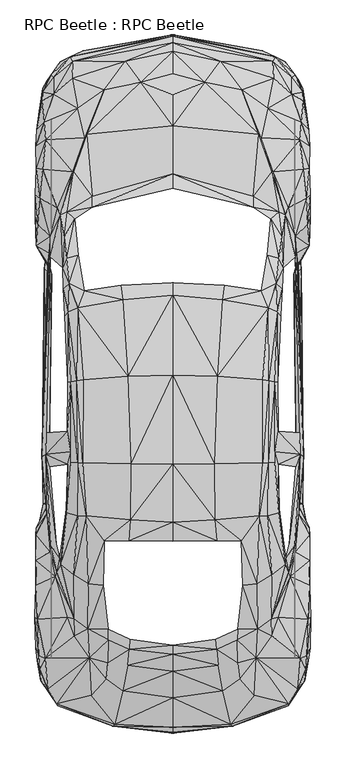
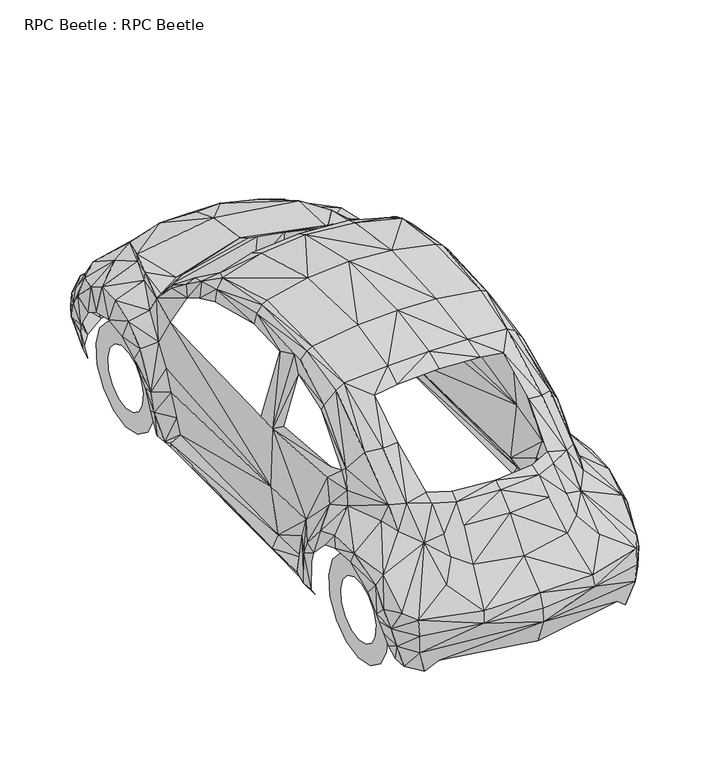
"""IFC4 building model written with IfcOpenShell, lengths in millimetres: proxy geometry, RPC Beetle : RPC Beetle."""

import ifcopenshell
import ifcopenshell.guid

model = None  # the IFC model being written
_history = None  # IfcOwnerHistory: only IFC2X3 demands one
_inside = {}  # id of a spatial element -> (the spatial element, [elements in it])
_under = {}  # id of a project, library or spatial element -> (it, [spatial elements below it])
_declared = {}  # id of a project -> (the project, [libraries it declares])
_typed = {}  # id of a type object -> (the type object, [elements of that type])
_made_of = {}  # id of a material, layer set ... -> (it, [elements and type objects made of it])


def new_model(schema):
    """Start an empty IFC model of exactly this schema.

    Asked for "IFC4X3", IfcOpenShell would pick the latest addendum, in which some entities
    have other attributes; the version numbers below select the first issue.
    IFC2X3 requires an IfcOwnerHistory on every rooted entity: one is made here for all.
    """
    global model, _history
    if schema == "IFC4X3":
        model = ifcopenshell.file(schema_version=(4, 3, 0, 0))
    else:
        model = ifcopenshell.file(schema=schema)
    _inside.clear()
    _under.clear()
    _declared.clear()
    _typed.clear()
    _made_of.clear()
    _history = None
    if model.schema == "IFC2X3":
        org = make("IfcOrganization", Name="unknown")
        user = make(
            "IfcPersonAndOrganization",
            ThePerson=make("IfcPerson", FamilyName="unknown"),
            TheOrganization=org,
        )
        app = make(
            "IfcApplication",
            ApplicationDeveloper=org,
            Version="unknown",
            ApplicationFullName="unknown",
            ApplicationIdentifier="unknown",
        )
        _history = make(
            "IfcOwnerHistory",
            OwningUser=user,
            OwningApplication=app,
            ChangeAction="ADDED",
            CreationDate=0,
        )
    return model


def make(cls, **values):
    """One entity of the class cls with the attributes given. An attribute that is None is left unset."""
    return model.create_entity(
        cls, **{name: value for name, value in values.items() if value is not None}
    )


def rooted(cls, **values):
    """An entity with a GlobalId (a new one), such as an element, a storey or a relation."""
    return make(cls, GlobalId=ifcopenshell.guid.new(), OwnerHistory=_history, **values)


def si_unit(unit_type, name, prefix=None):
    """IfcSIUnit, for example si_unit("LENGTHUNIT", "METRE", prefix="MILLI")."""
    return make("IfcSIUnit", UnitType=unit_type, Prefix=prefix, Name=name)


def assignment(units):
    """IfcUnitAssignment: the units of a project."""
    return None if units is None else make("IfcUnitAssignment", Units=units)


def point(xyz):
    """IfcCartesianPoint."""
    return None if xyz is None else make("IfcCartesianPoint", Coordinates=xyz)


def direction(xyz):
    """IfcDirection."""
    return None if xyz is None else make("IfcDirection", DirectionRatios=xyz)


def frame(location, z_axis=None, x_axis=None):
    """IfcAxis2Placement3D, a coordinate frame: its origin and axes. An axis left out is left unset."""
    return make(
        "IfcAxis2Placement3D",
        Location=point(location),
        Axis=direction(z_axis),
        RefDirection=direction(x_axis),
    )


def origin():
    """The frame at (0, 0, 0) with its axes left unset."""
    return frame((0.0, 0.0, 0.0))


def place(relative_to, where):
    """IfcLocalPlacement: puts the frame where relative to a parent placement (None: the world)."""
    return make(
        "IfcLocalPlacement", PlacementRelTo=relative_to, RelativePlacement=where
    )


def context(
    kind, dimensions, precision=None, world=None, true_north=None, identifier=None
):
    """IfcGeometricRepresentationContext, for example the 3D "Model" context."""
    return make(
        "IfcGeometricRepresentationContext",
        ContextIdentifier=identifier,
        ContextType=kind,
        CoordinateSpaceDimension=dimensions,
        Precision=precision,
        WorldCoordinateSystem=world,
        TrueNorth=true_north,
    )


def project(units=None, contexts=None):
    """IfcProject with its units and contexts."""
    return rooted(
        "IfcProject",
        Name="project",
        RepresentationContexts=contexts,
        UnitsInContext=assignment(units),
    )


def spatial(cls, under=None, at=None, **own):
    """A site, building, storey or space (cls), placed at a placement, below another one or the project."""
    s = rooted(cls, ObjectPlacement=at, **own)
    if under is not None:
        _under.setdefault(under.id(), (under, []))[1].append(s)
    return s


def point_list(points):
    """IfcCartesianPointList2D or 3D."""
    cls = (
        "IfcCartesianPointList2D" if len(points[0]) == 2 else "IfcCartesianPointList3D"
    )
    return make(cls, CoordList=points)


def triangles(points, corners, closed=None, point_numbers=None):
    """IfcTriangulatedFaceSet: each triangle names its three corners, points numbered from 1."""
    return make(
        "IfcTriangulatedFaceSet",
        Coordinates=point_list(points),
        Closed=closed,
        CoordIndex=corners,
        PnIndex=point_numbers,
    )


def shape(context_of_items, identifier, shape_type, items):
    """IfcShapeRepresentation: the items that make up one representation, for example the "Body"."""
    return make(
        "IfcShapeRepresentation",
        ContextOfItems=context_of_items,
        RepresentationIdentifier=identifier,
        RepresentationType=shape_type,
        Items=items,
    )


def source(mapping_origin, context_of_items, identifier, shape_type, items):
    """IfcRepresentationMap: a shape defined once, which mapped items show again and again."""
    return make(
        "IfcRepresentationMap",
        MappingOrigin=mapping_origin,
        MappedRepresentation=shape(context_of_items, identifier, shape_type, items),
    )


def transform(
    local_origin,
    x_axis=None,
    y_axis=None,
    z_axis=None,
    scale=None,
    scale2=None,
    scale3=None,
    uniform=True,
):
    """IfcCartesianTransformationOperator3D, or its non-uniform kind. x_axis, y_axis, z_axis: its Axis1, 2, 3."""
    if uniform:
        return make(
            "IfcCartesianTransformationOperator3D",
            Axis1=direction(x_axis),
            Axis2=direction(y_axis),
            LocalOrigin=point(local_origin),
            Scale=scale,
            Axis3=direction(z_axis),
        )
    return make(
        "IfcCartesianTransformationOperator3DnonUniform",
        Axis1=direction(x_axis),
        Axis2=direction(y_axis),
        LocalOrigin=point(local_origin),
        Scale=scale,
        Axis3=direction(z_axis),
        Scale2=scale2,
        Scale3=scale3,
    )


def mapped(mapping_source, mapping_target):
    """IfcMappedItem: shows the shape of a source again, moved by a transform."""
    return make(
        "IfcMappedItem", MappingSource=mapping_source, MappingTarget=mapping_target
    )


def made_of(thing, what):
    """Note that an element or type object is made of a material, layer set ...; save() writes the relation."""
    if what is not None:
        _made_of.setdefault(what.id(), (what, []))[1].append(thing)
    return thing


def element(
    cls,
    number,
    at=None,
    inside=None,
    cuts=None,
    type_object=None,
    material=None,
    context=None,
    identifier="Body",
    shape_type=None,
    held_by="IfcProductDefinitionShape",
    body=None,
    shapes=None,
    **own,
):
    """One element of the class cls, such as IfcWall. Its Tag is "e" and its number.

    at: its placement. inside: the storey or other place that contains it. cuts: it is an
    opening in that element (IfcRelVoidsElement). A single representation is given by context,
    identifier, shape_type and body (its items); several are given by shapes. held_by: the class
    of the entity that holds the representations. save() writes the other relations.
    """
    e = rooted(cls, Tag="e%d" % number, ObjectPlacement=at, **own)
    if body is not None:
        shapes = [shape(context, identifier, shape_type, body)]
    if shapes is not None:
        e.Representation = make(held_by, Representations=shapes)
    if inside is not None:
        _inside.setdefault(inside.id(), (inside, []))[1].append(e)
    if cuts is not None:
        rooted(
            "IfcRelVoidsElement", RelatingBuildingElement=cuts, RelatedOpeningElement=e
        )
    if type_object is not None:
        _typed.setdefault(type_object.id(), (type_object, []))[1].append(e)
    return made_of(e, material)


def aggregate(whole, parts):
    """IfcRelAggregates: a whole, such as a stair, and the parts it consists of."""
    return rooted("IfcRelAggregates", RelatingObject=whole, RelatedObjects=parts)


def save(model, path):
    """Write the relations noted so far, then the file.

    IfcRelAggregates (storeys below a building ...), IfcRelContainedInSpatialStructure (elements
    in a storey), IfcRelDefinesByType, IfcRelAssociatesMaterial and IfcRelDeclares: one each for
    every whole, place, type object, material and project.
    """
    for whole, parts in _under.values():
        aggregate(whole, parts)
    for where, things in _inside.values():
        rooted(
            "IfcRelContainedInSpatialStructure",
            RelatedElements=things,
            RelatingStructure=where,
        )
    for kind, things in _typed.values():
        rooted("IfcRelDefinesByType", RelatedObjects=things, RelatingType=kind)
    for what, things in _made_of.values():
        rooted("IfcRelAssociatesMaterial", RelatedObjects=things, RelatingMaterial=what)
    for by, libraries in _declared.values():
        rooted("IfcRelDeclares", RelatingContext=by, RelatedDefinitions=libraries)
    model.write(path)


def rpc_beetle_rpc_beetle_3ce7ba48(model_context):
    return source(origin(), model_context, "Body", "Tessellation", [
        triangles([(0.0, -748.5640469, 521.3893959), (0.0, -720.1452873, 603.6241656), (0.0, -696.6746996, 283.1362969), (0.0, -552.698168, 738.4050739), (0.0, -753.2493713, 438.4540149), (0.0, -253.6666567, 1039.7136446), (0.0, -401.102443, 921.3971746), (0.0, -304.8115909, 1012.258271), (0.0, 339.3168975, 1395.7139351), (0.0, 448.6129515, 1442.1297066), (0.0, 778.0774343, 1504.0465668), (0.0, 1285.0166222, 1509.4764679), (0.0, 1741.0736687, 1402.3260315), (0.0, 2430.9610645, 967.1999022), (0.0, 3130.000518, 632.0428888), (0.0, 3001.4374352, 771.5091579), (0.0, 2704.2451103, 928.7536297), (0.0, 3164.1993027, 220.1684652), (0.0, 2883.1647125, 858.7358105), (0.0, 3222.5253937, 395.8040382), (0.0, 3178.9995621, 555.7633515), (0.0, 3213.942778, 530.2784609), (-338.1784132, -715.5037102, 523.0095732), (-331.0408765, -702.1482754, 593.465229), (-244.7338081, -218.0228295, 1034.0649342), (-248.9812778, -275.9549947, 1002.9312967), (-257.7389736, -368.17353, 911.8512457), (-249.0688632, 342.8199903, 1381.001025), (-285.238149, -511.5369813, 760.4306917), (-240.1360146, 460.0855433, 1426.5848705), (-236.4577871, 780.8799522, 1493.4060825), (-652.4920767, -590.2248745, 370.4943186), (-540.0870918, -593.333878, 283.4428189), (-181.240518, 2954.2772324, 806.3210592), (-253.1849819, 1278.5798058, 1496.1646351), (-379.8650402, -444.3654636, 798.2639202), (-370.9321916, -353.3292326, 889.1688366), (-367.998359, -222.2265155, 1003.4567734), (-368.3924483, -160.7037083, 1036.6922447), (-390.1553278, 342.863774, 1359.0192272), (-282.5670547, 1713.2679531, 1399.3045589), (-397.3366482, 87.4893818, 1215.3492176), (-463.1069432, -537.7663033, 704.8193333), (-271.4885704, 3072.331073, 662.6947969), (-475.7618031, -323.0713775, 849.8467455), (-463.7199872, 3085.9052444, 214.2570165), (-482.2425121, 95.7654028, 1203.3949327), (-485.0449574, -159.3024857, 1005.0769506), (-568.7247334, 3071.4988564, 546.7429356), (-493.539933, 483.2496454, 1391.2912399), (-583.2625088, 3099.3922119, 522.0462235), (-510.267146, 3132.2774139, 369.3995816), (-391.8630724, 2911.6272194, 782.7628315), (-656.3454752, -597.8440679, 480.0968582), (-660.2426937, -584.8389024, 576.2563594), (-562.2878443, -200.0695467, 879.7105476), (-560.054623, -101.457906, 987.1674334), (-512.4565473, 786.1783207, 1448.435281), (-541.7948364, 484.782219, 1359.8511532), (-563.9955889, 148.5743069, 1172.3051153), (-608.4846974, -561.2369273, 218.4607206), (-511.2742793, 1258.5246346, 1456.1858253), (-542.4078804, 784.6895308, 1430.657151), (-458.8594554, 2304.0621243, 949.0276829), (-601.0406387, -92.7439938, 893.1973698), (-503.7426533, 1765.2887604, 1320.9670441), (-546.0423243, 1253.0072388, 1441.5166626), (-603.0111217, 501.1591264, 1278.5798058), (-580.1535416, 788.8931986, 1378.7239838), (-607.2148258, 519.8568223, 1235.1416142), (-601.2595934, 965.2732029, 1337.0374294), (-712.4823103, -503.0858256, 590.4876128), (-542.6706187, 1670.0487888, 1361.1648811), (-490.6061005, 2657.8729408, 893.5038918), (-599.6394161, 778.0774343, 1307.3049419), (-598.0630225, 1243.7240845, 1343.7807678), (-639.5744785, 208.1266312, 1062.483621), (-680.4291796, -470.2006599, 218.6796571), (-538.4669146, 1966.7157097, 1180.5811363), (-580.9855039, 1248.2342743, 1401.7567348), (-644.5225777, 243.2887836, 1028.2848364), (-502.3414307, 2635.8036484, 866.0046982), (-660.7243504, 162.2363182, 955.2456173), (-690.2377378, -396.5922532, 226.824309), (-559.1350571, 2175.0175301, 1011.1634977), (-670.1826393, 140.8675371, 872.7043619), (-662.4758423, 324.2974654, 1009.4557531), (-615.0967575, 1623.4577374, 1262.1152584), (-594.6475333, 1646.0964718, 1321.2735661), (-589.4366959, 1809.6026253, 1269.4280388), (-728.8153976, -481.9797738, 373.2091965), (-751.5854467, -454.4368329, 476.550018), (-694.047389, 315.3208331, 957.7853605), (-726.5821764, -327.3188653, 735.5588814), (-622.9348692, 1777.2429726, 1192.7981232), (-564.6524165, 2445.7178673, 934.1395655), (-731.7930502, -393.877339, 324.1222944), (-571.0017383, 2444.2728973, 884.1769175), (-698.6451462, 279.8521587, 807.6347145), (-604.2809933, 1949.7695057, 1170.4659834), (-587.4224293, 3013.0852707, 200.1133485), (-690.9384218, 574.2420928, 283.6179717), (-750.2279715, -381.0035608, 396.9863425), (-627.532699, 1896.2599812, 1124.7070759), (-602.4856813, 2215.5656364, 949.1590702), (-619.4318127, 2072.8151928, 1075.2698318), (-710.4680437, 549.6329844, 448.6129515), (-764.7219995, -360.335382, 467.5295657), (-699.5209648, 762.620093, 1015.4985529), (-763.3207769, -313.2189629, 670.9270706), (-757.8472012, -390.9435428, 564.6524165), (-717.4742294, 496.2985946, 583.5690308), (-722.7288506, 461.2240276, 180.9777796), (-717.6493641, 554.4496963, 179.8830608), (-771.4654106, -341.8128571, 511.011541), (-573.9355708, 2975.4707062, 682.6185808), (-730.7859169, 375.8802907, 185.1814656), (-541.1817924, 2805.3964943, 782.9379662), (-639.7496859, 2198.4442978, 944.2547184), (-738.9305506, 551.5596474, 222.4016865), (-781.5805635, -268.7736743, 609.2290924), (-772.2974092, -106.0556904, 755.9205019), (-721.7217173, 957.7416132, 967.0247675), (-703.3305433, 810.1306377, 292.3318839), (-724.8306845, 835.0462681, 964.3536369), (-757.7596338, 370.5381022, 225.46687), (-785.3463221, -89.9415304, 695.492359), (-779.6538643, 80.9211054, 675.5686478), (-779.3910896, 89.5036484, 754.6505939), (-760.3869444, 444.1027253, 223.1460814), (-778.0774343, 192.1000477, 630.9043682), (-658.6225164, 2237.1532722, 849.7591782), (-770.939934, 345.4910846, 426.1932444), (-774.1802885, 315.1456621, 501.684603), (-781.1864742, 232.2540829, 695.886521), (-719.2257214, 810.0868177, 185.8382933), (-689.8874685, 1858.8647346, 293.9082593), (-696.6746996, 1958.8775253, 956.4279579), (-779.7414316, 377.369117, 532.3802948), (-778.1212543, 416.9976574, 439.7238865), (-745.498827, 819.5889267, 613.6517149), (-677.7143017, 2884.8285645, 670.6205486), (-697.5504456, 2077.4130226, 756.8838152), (-639.6182985, 3069.1780678, 391.6879377), (-713.0077869, 1918.2417789, 536.7153863), (-718.1748407, 1909.8781906, 192.97583), (-705.1696753, 1981.9540237, 648.2884089), (-730.7859169, 1891.093, 233.3488017), (-673.9922178, 2907.8614609, 198.6683241), (-726.8886984, 2038.9229301, 189.9544119), (-721.6340773, 1973.3715534, 189.9544119), (-678.1959583, 2982.5644592, 540.5249648), (-699.6085321, 2815.6865639, 206.1999501), (-696.3681776, 2991.5851295, 517.4046464), (-723.6484165, 2624.6813622, 787.5795433), (-699.0830555, 1882.466637, 390.3742825), (-764.8971342, 2042.1632847, 362.5686032), (-741.7768158, 2457.6720795, 808.6855951), (-716.1605742, 2965.1367439, 449.5325174), (-766.4297441, 2001.1333763, 376.580902), (-731.5740955, 2724.4313782, 727.6331297), (-771.1588886, 2084.5942703, 482.2425121), (-759.1170364, 2291.4072281, 780.0917009), (-769.0132347, 2143.3146687, 699.0392355), (-777.5520304, 2022.8525448, 494.8098046), (-742.4774271, 2846.8640213, 601.8726374), (-782.1059675, 2185.6580143, 616.4541601), (-739.5435946, 2918.4145958, 427.3755486), (-741.1199518, 2896.5202927, 519.8130023), (-750.4031061, 2804.433181, 398.0810431), (-782.2373549, 2313.1701439, 680.7357016), (-778.0774343, 2462.7953133, 693.5219124), (-759.9052151, 2786.611013, 455.2250115), (-774.1802885, 2682.8324638, 602.660816), (-780.3544756, 2589.4317696, 666.3292408), (-742.6088144, 809.1235044, 220.3874017), (0.0, 2349.0766731, 1011.1634977), (-458.8594554, 2239.9557175, 1006.6095606), (0.0, 1812.0110538, 1368.2147415), (-293.952043, 1795.8092812, 1359.1506145), (-580.2411089, 849.7154308, 1381.7892036), (338.1784132, -715.5037102, 523.0095732), (331.0408765, -702.1482754, 593.465229), (244.7338081, -218.0228295, 1034.0649342), (248.9812778, -275.9549947, 1002.9312967), (257.7389736, -368.17353, 911.8512457), (249.0688632, 342.8199903, 1381.001025), (285.238149, -511.5369813, 760.4306917), (240.1360146, 460.0855433, 1426.5848705), (236.4577871, 780.8799522, 1493.4060825), (652.4920767, -590.2248745, 370.4943186), (540.0870918, -593.333878, 283.4428189), (181.240518, 2954.2772324, 806.3210592), (253.1849819, 1278.5798058, 1496.1646351), (379.8650402, -444.3654636, 798.2639202), (370.9321916, -353.3292326, 889.1688366), (367.998359, -222.2265155, 1003.4567734), (368.3924483, -160.7037083, 1036.6922447), (390.1553278, 342.863774, 1359.0192272), (282.5670547, 1713.2679531, 1399.3045589), (397.3366482, 87.4893818, 1215.3492176), (463.1069432, -537.7663033, 704.8193333), (271.4885704, 3072.331073, 662.6947969), (475.7618031, -323.0713775, 849.8467455), (463.7199872, 3085.9052444, 214.2570165), (482.2425121, 95.7654028, 1203.3949327), (485.0449574, -159.3024857, 1005.0769506), (568.7247334, 3071.4988564, 546.7429356), (493.539933, 483.2496454, 1391.2912399), (583.2625088, 3099.3922119, 522.0462235), (510.267146, 3132.2774139, 369.3995816), (391.8630724, 2911.6272194, 782.7628315), (656.3454752, -597.8440679, 480.0968582), (660.2426937, -584.8389024, 576.2563594), (562.2878443, -200.0695467, 879.7105476), (560.054623, -101.457906, 987.1674334), (512.4565473, 786.1783207, 1448.435281), (541.7948364, 484.782219, 1359.8511532), (563.9955889, 148.5743069, 1172.3051153), (608.4846974, -561.2369273, 218.4607206), (511.2742793, 1258.5246346, 1456.1858253), (542.4078804, 784.6895308, 1430.657151), (458.8594554, 2304.0621243, 949.0276829), (601.0406387, -92.7439938, 893.1973698), (503.7426533, 1765.2887604, 1320.9670441), (546.0423243, 1253.0072388, 1441.5166626), (603.0111217, 501.1591264, 1278.5798058), (580.1535416, 788.8931986, 1378.7239838), (607.2148258, 519.8568223, 1235.1416142), (601.2595934, 965.2732029, 1337.0374294), (712.4823103, -503.0858256, 590.4876128), (542.6706187, 1670.0487888, 1361.1648811), (490.6061005, 2657.8729408, 893.5038918), (599.6394161, 778.0774343, 1307.3049419), (598.0630225, 1243.7240845, 1343.7807678), (639.5744785, 208.1266312, 1062.483621), (680.4729269, -470.2006599, 218.6796571), (538.4669146, 1966.7157097, 1180.5811363), (580.9855039, 1248.2342743, 1401.7567348), (644.5225777, 243.2887836, 1028.2848364), (502.3414307, 2635.8036484, 866.0046982), (660.7243504, 162.2363182, 955.2456173), (690.2377378, -396.5922532, 226.824309), (559.1350571, 2175.0175301, 1011.1634977), (670.1826393, 140.8675371, 872.7043619), (662.4758423, 324.2974654, 1009.4557531), (615.0967575, 1623.4577374, 1262.1152584), (594.6475333, 1646.0964718, 1321.2735661), (589.4366959, 1809.6026253, 1269.4280388), (728.8153976, -481.9797738, 373.2091965), (751.5854467, -454.4368329, 476.550018), (694.047389, 315.3208331, 957.7853605), (726.5821764, -327.3188653, 735.5588814), (622.9348692, 1777.2429726, 1192.7981232), (564.6524165, 2445.7178673, 934.1395655), (731.7930502, -393.877339, 324.1222944), (571.0017383, 2444.2728973, 884.1769175), (698.6451462, 279.8521587, 807.6347145), (604.2809933, 1949.7695057, 1170.4659834), (587.4224293, 3013.0852707, 200.1133485), (690.9384218, 574.2420928, 283.6179717), (750.2279715, -381.0035608, 396.9863425), (627.532699, 1896.2599812, 1124.7070759), (602.4856813, 2215.5656364, 949.1590702), (619.4318127, 2072.8151928, 1075.2698318), (710.4680437, 549.6329844, 448.6129515), (764.7219995, -360.335382, 467.5295657), (699.5209648, 762.620093, 1015.4985529), (763.3207769, -313.2189629, 670.9270706), (757.8472012, -390.9435428, 564.6524165), (717.4742294, 496.2985946, 583.5690308), (722.7288506, 461.2240276, 180.9777796), (717.6493641, 554.4496963, 179.8830608), (771.4654106, -341.8128571, 511.011541), (573.9355708, 2975.4707062, 682.6185808), (730.7859169, 375.8802907, 185.1814656), (541.1817924, 2805.3964943, 782.9379662), (639.7496859, 2198.4442978, 944.2547184), (738.9305506, 551.5596474, 222.4016865), (781.5805635, -268.7736743, 609.2290924), (772.2974092, -106.0556904, 755.9205019), (721.7654646, 957.7416132, 967.0247675), (703.3305433, 810.1306377, 292.3318839), (724.8306845, 835.0462681, 964.3536369), (757.7596338, 370.5381022, 225.46687), (785.3463221, -89.9415304, 695.492359), (779.6538643, 80.9211054, 675.5686478), (779.4349096, 89.5036484, 754.6505939), (760.3869444, 444.1027253, 223.1460814), (778.0774343, 192.1000477, 630.9043682), (658.6225164, 2237.1532722, 849.7591782), (770.939934, 345.4910846, 426.1932444), (774.1802885, 315.1456621, 501.684603), (781.1864742, 232.2540829, 695.886521), (719.2257214, 810.0868177, 185.8382933), (689.8874685, 1858.8647346, 293.9082593), (696.6746996, 1958.8775253, 956.4279579), (779.7414316, 377.369117, 532.3802948), (778.1212543, 416.9976574, 439.7238865), (745.498827, 819.5889267, 613.6517149), (677.7143017, 2884.8285645, 670.6205486), (697.5504456, 2077.4130226, 756.8838152), (639.6182985, 3069.1780678, 391.6879377), (713.0077869, 1918.2417789, 536.7153863), (718.1748407, 1909.8781906, 192.97583), (705.1696753, 1981.9540237, 648.2884089), (730.7859169, 1891.093, 233.3488017), (673.9922178, 2907.8614609, 198.6683241), (726.8886984, 2038.9229301, 189.9544119), (721.6340773, 1973.3715534, 189.9544119), (678.1959583, 2982.5644592, 540.5249648), (699.6085321, 2815.6865639, 206.1999501), (696.3681776, 2991.5851295, 517.4046464), (723.6484165, 2624.6813622, 787.5795433), (699.0830555, 1882.466637, 390.3742825), (764.8971342, 2042.1632847, 362.5686032), (741.7768158, 2457.6720795, 808.6855951), (716.1605742, 2965.1367439, 449.5325174), (766.4297441, 2001.1333763, 376.580902), (731.5740955, 2724.4313782, 727.6331297), (771.202636, 2084.5942703, 482.2425121), (759.1170364, 2291.4072281, 780.0917009), (769.0132347, 2143.3146687, 699.0392355), (777.5520304, 2022.8525448, 494.8098046), (742.4774271, 2846.8640213, 601.8726374), (782.1059675, 2185.6580143, 616.4541601), (739.5435946, 2918.4145958, 427.3755486), (741.1199518, 2896.5202927, 519.8130023), (750.4031061, 2804.433181, 398.0810431), (782.2373549, 2313.1701439, 680.7357016), (778.0774343, 2462.7953133, 693.5219124), (759.9052151, 2786.611013, 455.2250115), (774.1802885, 2682.8324638, 602.660816), (780.3544756, 2589.4317696, 666.3292408), (742.6088144, 809.1235044, 220.3874017), (458.8594554, 2239.9557175, 1006.6095606), (293.952043, 1795.8092812, 1359.1506145), (580.2411089, 849.7154308, 1381.7892036), (-693.1715704, 2430.2605259, 0.0015107), (-693.1715704, 2430.2605259, 117.836303), (-693.1715704, 2557.1157188, 26.9752135), (-693.1715704, 2507.7661148, 134.3007686), (-693.1715704, 2661.9892593, 103.1671675), (-693.1715704, 2571.9162689, 180.8917202), (-693.1715704, 2726.8399521, 215.4846123), (-693.1715704, 2611.544664, 249.552046), (-693.1715704, 2740.4144142, 344.4416937), (-693.1715704, 2619.820903, 328.3713083), (-693.1715704, 2700.3479645, 467.7938301), (-693.1715704, 2595.3430367, 403.7312797), (-693.1715704, 2613.5590759, 564.1284659), (-693.1715704, 2542.3151688, 462.6267763), (-693.1715704, 2495.111364, 616.8935955), (-693.1715704, 2469.8890663, 494.898898), (-693.1715704, 2365.4098331, 616.8935955), (-693.1715704, 2390.6319855, 494.898898), (-693.1715704, 2246.9619759, 564.1284659), (-693.1715704, 2318.2057377, 462.6267763), (-693.1715704, 2160.1732327, 467.7938301), (-693.1715704, 2265.1780151, 403.7312797), (-693.1715704, 2120.1067829, 344.4416937), (-693.1715704, 2240.7001488, 328.3713083), (-693.1715704, 2133.6810997, 215.4846123), (-693.1715704, 2248.9762424, 249.552046), (-693.1715704, 2198.5319378, 103.1671675), (-693.1715704, 2288.6047829, 180.8917202), (-693.1715704, 2303.4053329, 26.9752135), (-693.1715704, 2352.754937, 134.3007686), (693.1715704, 2430.2605259, 0.0015107), (693.1715704, 2430.2605259, 117.836303), (693.1715704, 2303.4053329, 26.9752135), (693.1715704, 2352.754937, 134.3007686), (693.1715704, 2198.5319378, 103.1671675), (693.1715704, 2288.6047829, 180.8917202), (693.1715704, 2133.6810997, 215.4846123), (693.1715704, 2248.9762424, 249.552046), (693.1715704, 2120.1067829, 344.4416937), (693.1715704, 2240.7001488, 328.3713083), (693.1715704, 2160.1732327, 467.7938301), (693.1715704, 2265.1780151, 403.7312797), (693.1715704, 2246.9619759, 564.1284659), (693.1715704, 2318.2057377, 462.6267763), (693.1715704, 2365.4098331, 616.8935955), (693.1715704, 2390.6319855, 494.898898), (693.1715704, 2495.111364, 616.8935955), (693.1715704, 2469.8890663, 494.898898), (693.1715704, 2613.5590759, 564.1284659), (693.1715704, 2542.3151688, 462.6267763), (693.1715704, 2700.3479645, 467.7938301), (693.1715704, 2595.3430367, 403.7312797), (693.1715704, 2740.4144142, 344.4416937), (693.1715704, 2619.820903, 328.3713083), (693.1715704, 2726.8399521, 215.4846123), (693.1715704, 2611.544664, 249.552046), (693.1715704, 2661.9892593, 103.1671675), (693.1715704, 2571.9162689, 180.8917202), (693.1715704, 2557.1157188, 26.9752135), (693.1715704, 2507.7661148, 134.3007686), (-693.1715704, -13.5744281, 0.0015107), (-693.1715704, -13.5744281, 117.836303), (-693.1715704, 113.2807944, 26.9752135), (-693.1715704, 63.9311767, 134.3007686), (-693.1715704, 218.1541986, 103.1671675), (-693.1715704, 128.0812991, 180.8917202), (-693.1715704, 283.0049277, 215.4846123), (-693.1715704, 167.7098758, 249.552046), (-693.1715704, 296.5793535, 344.4416937), (-693.1715704, 175.9858968, 328.3713083), (-693.1715704, 256.5129038, 467.7938301), (-693.1715704, 151.5081304, 403.7312797), (-693.1715704, 169.7241424, 564.1284659), (-693.1715704, 98.4802897, 462.6267763), (-693.1715704, 51.2763078, 616.8935955), (-693.1715704, 26.0541442, 494.898898), (-693.1715704, -78.425164, 616.8935955), (-693.1715704, -53.2030025, 494.898898), (-693.1715704, -196.872994, 564.1284659), (-693.1715704, -125.6291413, 462.6267763), (-693.1715704, -283.6617554, 467.7938301), (-693.1715704, -178.6569911, 403.7312797), (-693.1715704, -323.7282051, 344.4416937), (-693.1715704, -203.1347484, 328.3713083), (-693.1715704, -310.1537793, 215.4846123), (-693.1715704, -194.8587274, 249.552046), (-693.1715704, -245.3030502, 103.1671675), (-693.1715704, -155.2301507, 180.8917202), (-693.1715704, -140.429646, 26.9752135), (-693.1715704, -91.0800329, 134.3007686), (693.1715704, -13.5744281, 0.0015107), (693.1715704, -13.5744281, 117.836303), (693.1715704, -140.429646, 26.9752135), (693.1715704, -91.0800329, 134.3007686), (693.1715704, -245.3030502, 103.1671675), (693.1715704, -155.2301507, 180.8917202), (693.1715704, -310.1537793, 215.4846123), (693.1715704, -194.8587274, 249.552046), (693.1715704, -323.7282051, 344.4416937), (693.1715704, -203.1347484, 328.3713083), (693.1715704, -283.6617554, 467.7938301), (693.1715704, -178.6569911, 403.7312797), (693.1715704, -196.872994, 564.1284659), (693.1715704, -125.6291413, 462.6267763), (693.1715704, -78.425164, 616.8935955), (693.1715704, -53.2030025, 494.898898), (693.1715704, 51.2763078, 616.8935955), (693.1715704, 26.0541442, 494.898898), (693.1715704, 169.7241424, 564.1284659), (693.1715704, 98.4802897, 462.6267763), (693.1715704, 256.5129038, 467.7938301), (693.1715704, 151.5081304, 403.7312797), (693.1715704, 296.5793535, 344.4416937), (693.1715704, 175.9858968, 328.3713083), (693.1715704, 283.0049277, 215.4846123), (693.1715704, 167.7098758, 249.552046), (693.1715704, 218.1541986, 103.1671675), (693.1715704, 128.0812991, 180.8917202), (693.1715704, 113.2807944, 26.9752135), (693.1715704, 63.9311767, 134.3007686)], [[67, 58, 62], [67, 63, 58], [53, 82, 74], [34, 17, 19], [118, 82, 53], [155, 98, 82], [155, 158, 98], [34, 74, 17], [172, 155, 175], [172, 158, 155], [159, 168, 169], [166, 142, 169], [175, 161, 174], [175, 155, 161], [142, 152, 169], [154, 169, 152], [160, 145, 165], [160, 156, 145], [162, 160, 165], [162, 157, 160], [34, 53, 74], [74, 96, 64], [82, 96, 74], [82, 98, 96], [36, 29, 27], [29, 43, 24], [23, 55, 54], [23, 24, 55], [23, 2, 24], [23, 1, 2], [5, 1, 23], [134, 140, 133], [134, 139, 140], [117, 130, 113], [117, 126, 130], [113, 120, 114], [113, 130, 120], [140, 112, 107], [140, 139, 112], [92, 108, 103], [91, 103, 97], [91, 92, 103], [61, 33, 32], [84, 78, 91], [84, 91, 97], [38, 26, 25], [77, 81, 83], [63, 50, 58], [63, 59, 50], [68, 63, 69], [68, 59, 63], [181, 75, 69], [74, 64, 17], [64, 14, 17], [64, 178, 14], [178, 177, 14], [34, 19, 16], [53, 34, 44], [21, 44, 15], [21, 49, 44], [44, 34, 15], [34, 16, 15], [22, 49, 21], [22, 51, 49], [20, 51, 22], [20, 52, 51], [18, 52, 20], [18, 46, 52], [51, 152, 49], [51, 154, 152], [101, 144, 46], [144, 52, 46], [101, 159, 144], [159, 169, 154], [101, 168, 159], [101, 149, 168], [149, 170, 168], [149, 153, 170], [168, 173, 169], [168, 170, 173], [49, 142, 116], [49, 152, 142], [49, 116, 44], [116, 142, 118], [161, 155, 118], [155, 82, 118], [142, 161, 118], [158, 132, 98], [158, 163, 132], [172, 163, 158], [172, 171, 163], [98, 119, 96], [98, 132, 119], [171, 164, 163], [171, 167, 164], [163, 143, 132], [163, 164, 143], [96, 105, 64], [96, 119, 105], [105, 178, 64], [105, 85, 178], [167, 165, 164], [167, 162, 165], [165, 143, 164], [165, 147, 143], [150, 160, 157], [150, 151, 160], [151, 156, 160], [151, 148, 137], [13, 35, 12], [13, 41, 35], [12, 31, 11], [12, 35, 31], [35, 58, 31], [35, 62, 58], [11, 30, 10], [11, 31, 30], [31, 50, 30], [31, 58, 50], [10, 28, 9], [10, 30, 28], [30, 40, 28], [30, 50, 40], [125, 75, 181], [125, 109, 75], [125, 87, 109], [125, 93, 87], [123, 141, 125], [137, 141, 156], [137, 124, 141], [148, 124, 137], [148, 176, 124], [146, 176, 148], [146, 136, 176], [141, 112, 125], [112, 93, 125], [112, 99, 93], [124, 112, 141], [124, 107, 112], [124, 102, 107], [176, 102, 124], [176, 120, 102], [136, 120, 176], [136, 114, 120], [47, 40, 50], [47, 42, 40], [48, 42, 47], [48, 39, 42], [57, 47, 60], [57, 48, 47], [60, 50, 59], [60, 47, 50], [59, 77, 60], [59, 68, 77], [77, 57, 60], [77, 83, 57], [70, 77, 68], [70, 81, 77], [75, 68, 69], [75, 70, 68], [26, 6, 25], [26, 8, 6], [27, 8, 26], [27, 7, 8], [29, 7, 27], [29, 4, 7], [24, 4, 29], [24, 2, 4], [32, 5, 23], [33, 5, 32], [33, 3, 5], [32, 23, 54], [55, 45, 72], [55, 24, 43], [99, 83, 93], [99, 86, 83], [135, 86, 99], [135, 129, 86], [131, 129, 135], [131, 128, 129], [93, 81, 87], [93, 83, 81], [128, 122, 129], [128, 127, 122], [122, 86, 129], [122, 65, 86], [86, 57, 83], [86, 65, 57], [127, 110, 122], [127, 121, 110], [110, 94, 122], [122, 94, 65], [94, 56, 65], [56, 57, 65], [56, 48, 57], [56, 45, 48], [94, 45, 56], [115, 110, 121], [115, 111, 110], [111, 94, 110], [111, 72, 94], [108, 92, 115], [92, 111, 115], [78, 32, 91], [78, 61, 32], [45, 38, 48], [45, 37, 38], [37, 26, 38], [37, 27, 26], [36, 27, 37], [134, 135, 139], [134, 131, 135], [139, 99, 112], [139, 135, 99], [126, 140, 130], [126, 133, 140], [130, 107, 120], [130, 140, 107], [120, 107, 102], [45, 36, 37], [92, 55, 72], [92, 54, 55], [91, 54, 92], [91, 32, 54], [92, 72, 111], [72, 45, 94], [43, 45, 55], [43, 36, 45], [43, 29, 36], [79, 90, 66], [79, 100, 90], [90, 73, 66], [85, 100, 79], [85, 106, 100], [85, 105, 106], [105, 119, 106], [95, 88, 89], [90, 89, 73], [89, 67, 73], [73, 67, 62], [89, 76, 80], [89, 80, 67], [88, 76, 89], [73, 35, 41], [73, 62, 35], [69, 63, 181], [80, 63, 67], [76, 71, 80], [146, 148, 151], [141, 147, 145], [151, 137, 156], [173, 166, 169], [173, 174, 166], [166, 174, 161], [166, 161, 142], [52, 144, 51], [144, 154, 51], [144, 159, 154], [116, 53, 44], [116, 118, 53], [119, 143, 138], [143, 119, 132], [143, 147, 138], [138, 104, 119], [119, 104, 106], [104, 100, 106], [104, 90, 100], [104, 95, 90], [95, 89, 90], [25, 39, 38], [38, 39, 48], [141, 138, 147], [156, 141, 145], [165, 145, 147], [41, 179, 180], [41, 13, 179], [66, 41, 180], [66, 73, 41], [123, 125, 71], [125, 181, 71], [71, 181, 80], [181, 63, 80], [138, 141, 123], [226, 221, 217], [226, 217, 222], [212, 233, 241], [193, 19, 17], [277, 212, 241], [314, 241, 257], [314, 257, 317], [193, 17, 233], [331, 334, 314], [331, 314, 317], [318, 328, 327], [325, 328, 301], [334, 333, 320], [334, 320, 314], [301, 328, 311], [313, 311, 328], [319, 324, 304], [319, 304, 315], [321, 324, 319], [321, 319, 316], [193, 233, 212], [233, 223, 255], [241, 233, 255], [241, 255, 257], [195, 186, 188], [188, 183, 202], [182, 213, 214], [182, 214, 183], [182, 183, 2], [182, 2, 1], [5, 182, 1], [293, 292, 299], [293, 299, 298], [276, 272, 289], [276, 289, 285], [272, 273, 279], [272, 279, 289], [299, 266, 271], [299, 271, 298], [251, 262, 267], [250, 256, 262], [250, 262, 251], [220, 191, 192], [243, 250, 237], [243, 256, 250], [197, 184, 185], [236, 242, 240], [222, 217, 209], [222, 209, 218], [227, 228, 222], [227, 222, 218], [338, 228, 234], [233, 17, 223], [223, 17, 14], [223, 14, 336], [336, 14, 177], [193, 16, 19], [212, 203, 193], [21, 15, 203], [21, 203, 208], [203, 15, 193], [193, 15, 16], [22, 21, 208], [22, 208, 210], [20, 22, 210], [20, 210, 211], [18, 20, 211], [18, 211, 205], [210, 208, 311], [210, 311, 313], [260, 205, 303], [303, 205, 211], [260, 303, 318], [318, 313, 328], [260, 318, 327], [260, 327, 308], [308, 327, 329], [308, 329, 312], [327, 328, 332], [327, 332, 329], [208, 275, 301], [208, 301, 311], [208, 203, 275], [275, 277, 301], [320, 277, 314], [314, 277, 241], [301, 277, 320], [317, 257, 291], [317, 291, 322], [331, 317, 322], [331, 322, 330], [257, 255, 278], [257, 278, 291], [330, 322, 323], [330, 323, 326], [322, 291, 302], [322, 302, 323], [255, 223, 264], [255, 264, 278], [264, 223, 336], [264, 336, 244], [326, 323, 324], [326, 324, 321], [324, 323, 302], [324, 302, 306], [309, 316, 319], [309, 319, 310], [310, 319, 315], [310, 296, 307], [13, 12, 194], [13, 194, 200], [12, 11, 190], [12, 190, 194], [194, 190, 217], [194, 217, 221], [11, 10, 189], [11, 189, 190], [190, 189, 209], [190, 209, 217], [10, 9, 187], [10, 187, 189], [189, 187, 199], [189, 199, 209], [284, 338, 234], [284, 234, 268], [284, 268, 246], [284, 246, 252], [282, 284, 300], [296, 315, 300], [296, 300, 283], [307, 296, 283], [307, 283, 335], [305, 307, 335], [305, 335, 295], [300, 284, 271], [271, 284, 252], [271, 252, 258], [283, 300, 271], [283, 271, 266], [283, 266, 261], [335, 283, 261], [335, 261, 279], [295, 335, 279], [295, 279, 273], [206, 209, 199], [206, 199, 201], [207, 206, 201], [207, 201, 198], [216, 219, 206], [216, 206, 207], [219, 218, 209], [219, 209, 206], [218, 219, 236], [218, 236, 227], [236, 219, 216], [236, 216, 242], [229, 227, 236], [229, 236, 240], [234, 228, 227], [234, 227, 229], [185, 184, 6], [185, 6, 8], [186, 185, 8], [186, 8, 7], [188, 186, 7], [188, 7, 4], [183, 188, 4], [183, 4, 2], [191, 182, 5], [192, 191, 5], [192, 5, 3], [191, 213, 182], [214, 231, 204], [214, 202, 183], [258, 252, 242], [258, 242, 245], [294, 258, 245], [294, 245, 288], [290, 294, 288], [290, 288, 287], [252, 246, 240], [252, 240, 242], [287, 288, 281], [287, 281, 286], [281, 288, 245], [281, 245, 224], [245, 242, 216], [245, 216, 224], [286, 281, 269], [286, 269, 280], [269, 281, 253], [281, 224, 253], [253, 224, 215], [215, 224, 216], [215, 216, 207], [215, 207, 204], [253, 215, 204], [274, 280, 269], [274, 269, 270], [270, 269, 253], [270, 253, 231], [267, 274, 251], [251, 274, 270], [237, 250, 191], [237, 191, 220], [204, 207, 197], [204, 197, 196], [196, 197, 185], [196, 185, 186], [195, 196, 186], [293, 298, 294], [293, 294, 290], [298, 271, 258], [298, 258, 294], [285, 289, 299], [285, 299, 292], [289, 279, 266], [289, 266, 299], [279, 261, 266], [204, 196, 195], [251, 231, 214], [251, 214, 213], [250, 251, 213], [250, 213, 191], [251, 270, 231], [231, 253, 204], [202, 214, 204], [202, 204, 195], [202, 195, 188], [238, 225, 249], [238, 249, 259], [249, 225, 232], [244, 238, 259], [244, 259, 265], [244, 265, 264], [264, 265, 278], [254, 248, 247], [249, 232, 248], [248, 232, 226], [232, 221, 226], [248, 239, 235], [248, 226, 239], [247, 248, 235], [232, 200, 194], [232, 194, 221], [228, 338, 222], [239, 226, 222], [235, 239, 230], [305, 310, 307], [300, 304, 306], [310, 315, 296], [332, 328, 325], [332, 325, 333], [325, 320, 333], [325, 301, 320], [211, 210, 303], [303, 210, 313], [303, 313, 318], [275, 203, 212], [275, 212, 277], [278, 297, 302], [302, 291, 278], [302, 297, 306], [297, 278, 263], [278, 265, 263], [263, 265, 259], [263, 259, 249], [263, 249, 254], [254, 249, 248], [184, 197, 198], [197, 207, 198], [300, 306, 297], [315, 304, 300], [324, 306, 304], [200, 337, 179], [200, 179, 13], [225, 337, 200], [225, 200, 232], [282, 230, 284], [284, 230, 338], [230, 239, 338], [338, 239, 222], [297, 282, 300], [339, 342, 341], [339, 340, 342], [341, 344, 343], [341, 342, 344], [343, 346, 345], [343, 344, 346], [345, 348, 347], [345, 346, 348], [347, 350, 349], [347, 348, 350], [349, 352, 351], [349, 350, 352], [351, 354, 353], [351, 352, 354], [353, 356, 355], [353, 354, 356], [355, 358, 357], [355, 356, 358], [357, 360, 359], [357, 358, 360], [359, 362, 361], [359, 360, 362], [361, 364, 363], [361, 362, 364], [363, 366, 365], [363, 364, 366], [365, 368, 367], [365, 366, 368], [367, 340, 339], [367, 368, 340], [369, 372, 371], [369, 370, 372], [371, 374, 373], [371, 372, 374], [373, 376, 375], [373, 374, 376], [375, 378, 377], [375, 376, 378], [377, 380, 379], [377, 378, 380], [379, 382, 381], [379, 380, 382], [381, 384, 383], [381, 382, 384], [383, 386, 385], [383, 384, 386], [385, 388, 387], [385, 386, 388], [387, 390, 389], [387, 388, 390], [389, 392, 391], [389, 390, 392], [391, 394, 393], [391, 392, 394], [393, 396, 395], [393, 394, 396], [395, 398, 397], [395, 396, 398], [397, 370, 369], [397, 398, 370], [399, 402, 401], [399, 400, 402], [401, 404, 403], [401, 402, 404], [403, 406, 405], [403, 404, 406], [405, 408, 407], [405, 406, 408], [407, 410, 409], [407, 408, 410], [409, 412, 411], [409, 410, 412], [411, 414, 413], [411, 412, 414], [413, 416, 415], [413, 414, 416], [415, 418, 417], [415, 416, 418], [417, 420, 419], [417, 418, 420], [419, 422, 421], [419, 420, 422], [421, 424, 423], [421, 422, 424], [423, 426, 425], [423, 424, 426], [425, 428, 427], [425, 426, 428], [427, 400, 399], [427, 428, 400], [429, 432, 431], [429, 430, 432], [431, 434, 433], [431, 432, 434], [433, 436, 435], [433, 434, 436], [435, 438, 437], [435, 436, 438], [437, 440, 439], [437, 438, 440], [439, 442, 441], [439, 440, 442], [441, 444, 443], [441, 442, 444], [443, 446, 445], [443, 444, 446], [445, 448, 447], [445, 446, 448], [447, 450, 449], [447, 448, 450], [449, 452, 451], [449, 450, 452], [451, 454, 453], [451, 452, 454], [453, 456, 455], [453, 454, 456], [455, 458, 457], [455, 456, 458], [457, 430, 429], [457, 458, 430]], closed=False),
    ])


if __name__ == "__main__":
    model = new_model("IFC4")
    model_context = context("Model", 3, world=origin())
    ifc_project = project(units=[si_unit("LENGTHUNIT", "METRE", prefix="MILLI")], contexts=[model_context])
    site = spatial("IfcSite", under=ifc_project)
    building = spatial("IfcBuilding", under=site)
    placement = place(None, origin())
    rpc_beetle_rpc_beetle_shape = rpc_beetle_rpc_beetle_3ce7ba48(model_context)
    element("IfcBuildingElementProxy", 1, Name="RPC Beetle : RPC Beetle", ObjectType="RPC Beetle : RPC Beetle", at=placement, inside=building, context=model_context, shape_type="MappedRepresentation", body=[
        mapped(rpc_beetle_rpc_beetle_shape, transform((0.0, 0.0, 0.0), x_axis=(1.0, 0.0, 0.0), y_axis=(0.0, 1.0, 0.0), z_axis=(0.0, 0.0, 1.0))),
    ])
    save(model, "model.ifc")

# Revit data of these elements
# Type "RPC Beetle : RPC Beetle"
#   built-in parameter 1005195 = "RPC-16-0U6E-L4EG-ENH1-J3KF-SVEL-0TX4-C0"
#   Height = 0
